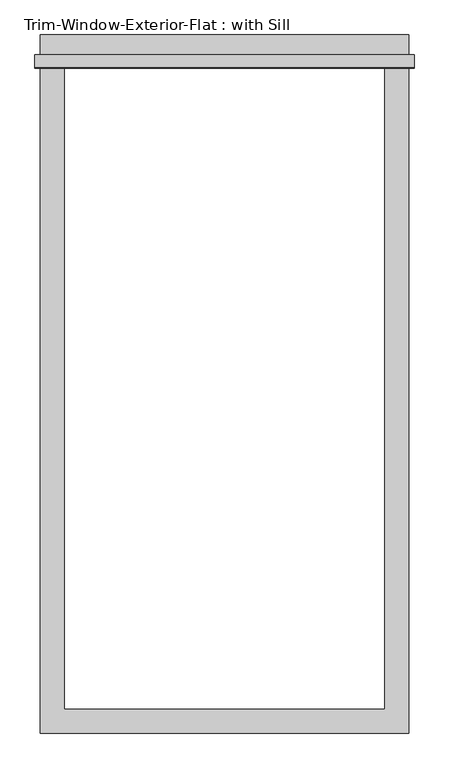
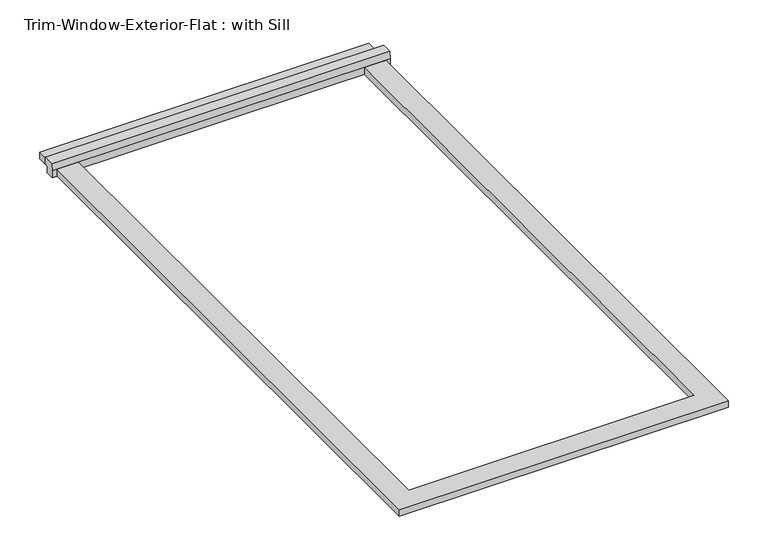
"""IFC4 building model written with IfcOpenShell, lengths in millimetres: proxy geometry, Trim-Window-Exterior-Flat : with Sill."""

from ifc_helpers import new_model, si_unit, frame, origin, origin_with_axes, place, context, project, spatial, polyline, outline, extrude, source, transform, mapped, element, save


def trim_window_exterior_flat_with_sill_a54b5ee7(model_context):
    return source(origin(), model_context, "Body", "SweptSolid", [
        extrude(outline(polyline([(438.15, 1546.1823709), (-438.15, 1546.1823709), (-438.15, 1603.3323709), (438.15, 1603.3323709), (438.15, 1546.1823709)])), origin_with_axes(), (0.0, 0.0, 1.0), 19.05),
        extrude(outline(polyline([(1555.75, 38.1), (1555.75, 19.05), (1546.1823709, 19.05), (1546.1823709, 0.0), (1524.0, 0.0), (1524.0, 19.05), (1526.4580645, 38.1), (1555.75, 38.1)])), frame((-450.85, 0.0, 0.0), z_axis=(1.0, 0.0, 0.0), x_axis=(0.0, 1.0, 0.0)), (0.0, 0.0, 1.0), 901.7),
        extrude(outline(polyline([(-438.15, -57.15), (-438.15, 1524.0), (-381.0, 1524.0), (-381.0, 0.0), (381.0, 0.0), (381.0, 1524.0), (438.15, 1524.0), (438.15, -57.15), (-438.15, -57.15)])), origin_with_axes(), (0.0, 0.0, 1.0), 19.05),
    ])


if __name__ == "__main__":
    model = new_model("IFC4")
    model_context = context("Model", 3, world=origin())
    ifc_project = project(units=[si_unit("LENGTHUNIT", "METRE", prefix="MILLI")], contexts=[model_context])
    site = spatial("IfcSite", under=ifc_project)
    building = spatial("IfcBuilding", under=site)
    placement = place(None, origin())
    trim_window_exterior_flat_with_sill_shape = trim_window_exterior_flat_with_sill_a54b5ee7(model_context)
    element("IfcBuildingElementProxy", 1, Name="Trim-Window-Exterior-Flat : with Sill", ObjectType="Trim-Window-Exterior-Flat : with Sill", at=placement, inside=building, context=model_context, shape_type="MappedRepresentation", body=[
        mapped(trim_window_exterior_flat_with_sill_shape, transform((0.0, 0.0, 0.0), x_axis=(1.0, 0.0, 0.0), y_axis=(0.0, 1.0, 0.0), z_axis=(0.0, 0.0, 1.0))),
    ])
    save(model, "model.ifc")

# Revit data of these elements
# Type "Trim-Window-Exterior-Flat : with Sill"
#   Trim Width = 0' - 2 1/4"
#   Trim Thickness_Picture Frame = 0' - 1 1/4"
#   Trim Thickness_with Sill = 0' - 0 3/4"
#   Sill Thickness = 0' - 1 1/4"
#   Opening Width [instance default] = 2' - 0"
#   Opening Height [instance default] = 3' - 0"
#   Default Elevation = 4' - 0"
#   Sill = yes
#   Picture Frame = no
#   Trim Material [instance default] = none
# Element 1 (IfcBuildingElementProxy, "Trim-Window-Exterior-Flat : with Sill")
#   Opening Width = 2' - 6"
#   Opening Height = 5' - 0"
#   Trim Material = Clad - White
#   Materials on its faces: "Clad - White"
# Materials
#   "Clad - White": class "Wood", colour RGB 242 242 238, transparency 0, Cost = 0
